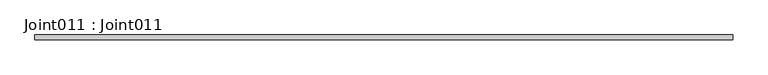
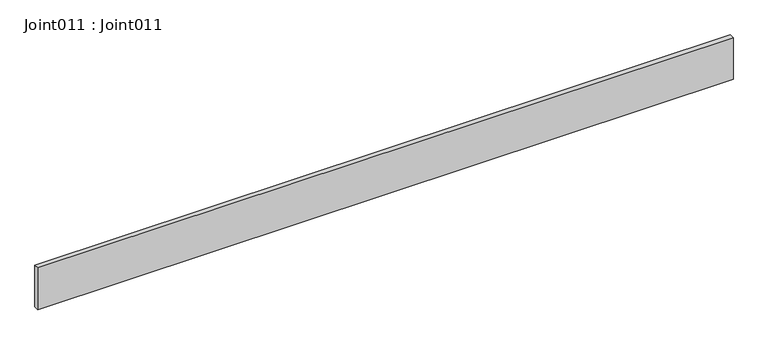
"""IFC4 building model written with IfcOpenShell, lengths in millimetres: proxy geometry, Joint011 : Joint011."""

from ifc_helpers import new_model, si_unit, frame, origin, place, context, project, spatial, polyline, outline, extrude, source, transform, mapped, element, save


def joint011_joint011_2a0334aa(model_context):
    return source(origin(), model_context, "Body", "SweptSolid", [
        extrude(outline(polyline([(14383.0178845, -4637.5417972), (14383.0178845, -4651.5044925), (12383.0178845, -4651.5044925), (12383.0178845, -4637.5417972), (14383.0178845, -4637.5417972)])), frame((0.0, 0.0, 36175.6882407), z_axis=(0.0, 0.0, 1.0), x_axis=(1.0, 0.0, 0.0)), (0.0, 0.0, 1.0), 127.0),
    ])


if __name__ == "__main__":
    model = new_model("IFC4")
    model_context = context("Model", 3, world=origin())
    ifc_project = project(units=[si_unit("LENGTHUNIT", "METRE", prefix="MILLI")], contexts=[model_context])
    site = spatial("IfcSite", under=ifc_project)
    building = spatial("IfcBuilding", under=site)
    placement = place(None, origin())
    joint011_joint011_shape = joint011_joint011_2a0334aa(model_context)
    element("IfcBuildingElementProxy", 1, Name="Joint011 : Joint011", ObjectType="Joint011 : Joint011", at=placement, inside=building, context=model_context, shape_type="MappedRepresentation", body=[
        mapped(joint011_joint011_shape, transform((0.0, 0.0, 0.0), x_axis=(1.0, 0.0, 0.0), y_axis=(0.0, 1.0, 0.0), z_axis=(0.0, 0.0, 1.0))),
    ])
    save(model, "model.ifc")

# Revit data of these elements
# Type "Joint011 : Joint011"
#   NameOverride = "Joint011"
# Element 1 (IfcBuildingElementProxy, "Joint011 : Joint011")
#   Materials on its faces: "CONCRETE EXPANSION JOINT - MINERAL FIBER"
# Materials
#   "CONCRETE EXPANSION JOINT - MINERAL FIBER": class "Unassigned", colour RGB 82 203 28, transparency 0
